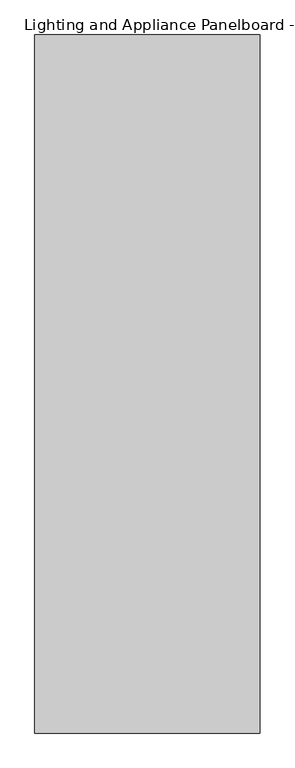
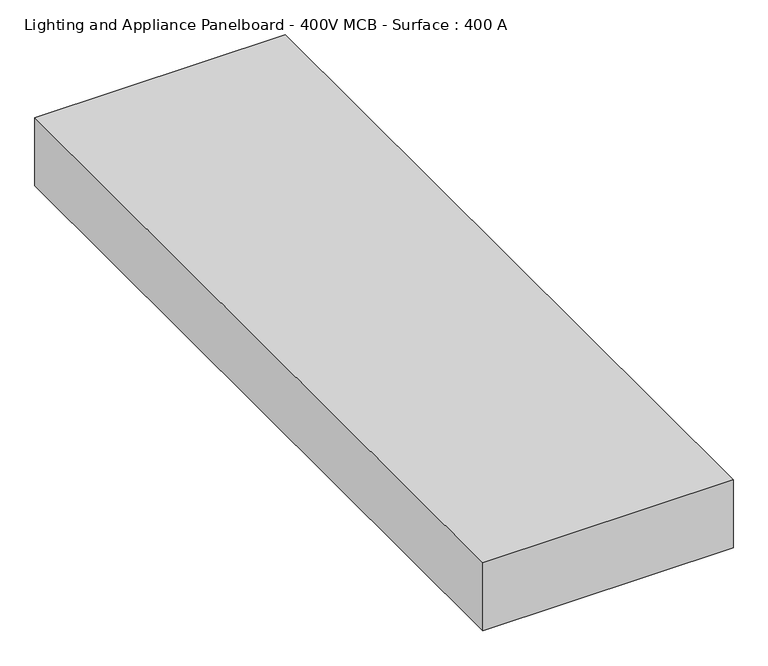
"""IFC4 building model written with IfcOpenShell, lengths in millimetres: proxy geometry, Lighting and Appliance Panelboard - 400V MCB - Surface : 400 A."""

import ifcopenshell
import ifcopenshell.guid

model = None  # the IFC model being written
_history = None  # IfcOwnerHistory: only IFC2X3 demands one
_inside = {}  # id of a spatial element -> (the spatial element, [elements in it])
_under = {}  # id of a project, library or spatial element -> (it, [spatial elements below it])
_declared = {}  # id of a project -> (the project, [libraries it declares])
_typed = {}  # id of a type object -> (the type object, [elements of that type])
_made_of = {}  # id of a material, layer set ... -> (it, [elements and type objects made of it])


def new_model(schema):
    """Start an empty IFC model of exactly this schema.

    Asked for "IFC4X3", IfcOpenShell would pick the latest addendum, in which some entities
    have other attributes; the version numbers below select the first issue.
    IFC2X3 requires an IfcOwnerHistory on every rooted entity: one is made here for all.
    """
    global model, _history
    if schema == "IFC4X3":
        model = ifcopenshell.file(schema_version=(4, 3, 0, 0))
    else:
        model = ifcopenshell.file(schema=schema)
    _inside.clear()
    _under.clear()
    _declared.clear()
    _typed.clear()
    _made_of.clear()
    _history = None
    if model.schema == "IFC2X3":
        org = make("IfcOrganization", Name="unknown")
        user = make(
            "IfcPersonAndOrganization",
            ThePerson=make("IfcPerson", FamilyName="unknown"),
            TheOrganization=org,
        )
        app = make(
            "IfcApplication",
            ApplicationDeveloper=org,
            Version="unknown",
            ApplicationFullName="unknown",
            ApplicationIdentifier="unknown",
        )
        _history = make(
            "IfcOwnerHistory",
            OwningUser=user,
            OwningApplication=app,
            ChangeAction="ADDED",
            CreationDate=0,
        )
    return model


def make(cls, **values):
    """One entity of the class cls with the attributes given. An attribute that is None is left unset."""
    return model.create_entity(
        cls, **{name: value for name, value in values.items() if value is not None}
    )


def rooted(cls, **values):
    """An entity with a GlobalId (a new one), such as an element, a storey or a relation."""
    return make(cls, GlobalId=ifcopenshell.guid.new(), OwnerHistory=_history, **values)


def si_unit(unit_type, name, prefix=None):
    """IfcSIUnit, for example si_unit("LENGTHUNIT", "METRE", prefix="MILLI")."""
    return make("IfcSIUnit", UnitType=unit_type, Prefix=prefix, Name=name)


def assignment(units):
    """IfcUnitAssignment: the units of a project."""
    return None if units is None else make("IfcUnitAssignment", Units=units)


def point(xyz):
    """IfcCartesianPoint."""
    return None if xyz is None else make("IfcCartesianPoint", Coordinates=xyz)


def direction(xyz):
    """IfcDirection."""
    return None if xyz is None else make("IfcDirection", DirectionRatios=xyz)


def frame(location, z_axis=None, x_axis=None):
    """IfcAxis2Placement3D, a coordinate frame: its origin and axes. An axis left out is left unset."""
    return make(
        "IfcAxis2Placement3D",
        Location=point(location),
        Axis=direction(z_axis),
        RefDirection=direction(x_axis),
    )


def origin():
    """The frame at (0, 0, 0) with its axes left unset."""
    return frame((0.0, 0.0, 0.0))


def origin_with_axes():
    """The frame at (0, 0, 0) with the z axis (0, 0, 1) and the x axis (1, 0, 0) written out."""
    return frame((0.0, 0.0, 0.0), z_axis=(0.0, 0.0, 1.0), x_axis=(1.0, 0.0, 0.0))


def place(relative_to, where):
    """IfcLocalPlacement: puts the frame where relative to a parent placement (None: the world)."""
    return make(
        "IfcLocalPlacement", PlacementRelTo=relative_to, RelativePlacement=where
    )


def context(
    kind, dimensions, precision=None, world=None, true_north=None, identifier=None
):
    """IfcGeometricRepresentationContext, for example the 3D "Model" context."""
    return make(
        "IfcGeometricRepresentationContext",
        ContextIdentifier=identifier,
        ContextType=kind,
        CoordinateSpaceDimension=dimensions,
        Precision=precision,
        WorldCoordinateSystem=world,
        TrueNorth=true_north,
    )


def project(units=None, contexts=None):
    """IfcProject with its units and contexts."""
    return rooted(
        "IfcProject",
        Name="project",
        RepresentationContexts=contexts,
        UnitsInContext=assignment(units),
    )


def spatial(cls, under=None, at=None, **own):
    """A site, building, storey or space (cls), placed at a placement, below another one or the project."""
    s = rooted(cls, ObjectPlacement=at, **own)
    if under is not None:
        _under.setdefault(under.id(), (under, []))[1].append(s)
    return s


def polyline(points):
    """IfcPolyline through the points."""
    return make("IfcPolyline", Points=[point(p) for p in points])


def outline(outer, holes=None, kind="AREA"):
    """IfcArbitraryClosedProfileDef: a profile drawn as a closed curve; with holes, ...WithVoids."""
    if holes is None:
        return make("IfcArbitraryClosedProfileDef", ProfileType=kind, OuterCurve=outer)
    return make(
        "IfcArbitraryProfileDefWithVoids",
        ProfileType=kind,
        OuterCurve=outer,
        InnerCurves=holes,
    )


def extrude(swept, where, along, depth):
    """IfcExtrudedAreaSolid: the profile swept, set in the frame where, extruded along a direction by depth."""
    return make(
        "IfcExtrudedAreaSolid",
        SweptArea=swept,
        Position=where,
        ExtrudedDirection=direction(along),
        Depth=depth,
    )


def shape(context_of_items, identifier, shape_type, items):
    """IfcShapeRepresentation: the items that make up one representation, for example the "Body"."""
    return make(
        "IfcShapeRepresentation",
        ContextOfItems=context_of_items,
        RepresentationIdentifier=identifier,
        RepresentationType=shape_type,
        Items=items,
    )


def source(mapping_origin, context_of_items, identifier, shape_type, items):
    """IfcRepresentationMap: a shape defined once, which mapped items show again and again."""
    return make(
        "IfcRepresentationMap",
        MappingOrigin=mapping_origin,
        MappedRepresentation=shape(context_of_items, identifier, shape_type, items),
    )


def transform(
    local_origin,
    x_axis=None,
    y_axis=None,
    z_axis=None,
    scale=None,
    scale2=None,
    scale3=None,
    uniform=True,
):
    """IfcCartesianTransformationOperator3D, or its non-uniform kind. x_axis, y_axis, z_axis: its Axis1, 2, 3."""
    if uniform:
        return make(
            "IfcCartesianTransformationOperator3D",
            Axis1=direction(x_axis),
            Axis2=direction(y_axis),
            LocalOrigin=point(local_origin),
            Scale=scale,
            Axis3=direction(z_axis),
        )
    return make(
        "IfcCartesianTransformationOperator3DnonUniform",
        Axis1=direction(x_axis),
        Axis2=direction(y_axis),
        LocalOrigin=point(local_origin),
        Scale=scale,
        Axis3=direction(z_axis),
        Scale2=scale2,
        Scale3=scale3,
    )


def mapped(mapping_source, mapping_target):
    """IfcMappedItem: shows the shape of a source again, moved by a transform."""
    return make(
        "IfcMappedItem", MappingSource=mapping_source, MappingTarget=mapping_target
    )


def made_of(thing, what):
    """Note that an element or type object is made of a material, layer set ...; save() writes the relation."""
    if what is not None:
        _made_of.setdefault(what.id(), (what, []))[1].append(thing)
    return thing


def element(
    cls,
    number,
    at=None,
    inside=None,
    cuts=None,
    type_object=None,
    material=None,
    context=None,
    identifier="Body",
    shape_type=None,
    held_by="IfcProductDefinitionShape",
    body=None,
    shapes=None,
    **own,
):
    """One element of the class cls, such as IfcWall. Its Tag is "e" and its number.

    at: its placement. inside: the storey or other place that contains it. cuts: it is an
    opening in that element (IfcRelVoidsElement). A single representation is given by context,
    identifier, shape_type and body (its items); several are given by shapes. held_by: the class
    of the entity that holds the representations. save() writes the other relations.
    """
    e = rooted(cls, Tag="e%d" % number, ObjectPlacement=at, **own)
    if body is not None:
        shapes = [shape(context, identifier, shape_type, body)]
    if shapes is not None:
        e.Representation = make(held_by, Representations=shapes)
    if inside is not None:
        _inside.setdefault(inside.id(), (inside, []))[1].append(e)
    if cuts is not None:
        rooted(
            "IfcRelVoidsElement", RelatingBuildingElement=cuts, RelatedOpeningElement=e
        )
    if type_object is not None:
        _typed.setdefault(type_object.id(), (type_object, []))[1].append(e)
    return made_of(e, material)


def aggregate(whole, parts):
    """IfcRelAggregates: a whole, such as a stair, and the parts it consists of."""
    return rooted("IfcRelAggregates", RelatingObject=whole, RelatedObjects=parts)


def save(model, path):
    """Write the relations noted so far, then the file.

    IfcRelAggregates (storeys below a building ...), IfcRelContainedInSpatialStructure (elements
    in a storey), IfcRelDefinesByType, IfcRelAssociatesMaterial and IfcRelDeclares: one each for
    every whole, place, type object, material and project.
    """
    for whole, parts in _under.values():
        aggregate(whole, parts)
    for where, things in _inside.values():
        rooted(
            "IfcRelContainedInSpatialStructure",
            RelatedElements=things,
            RelatingStructure=where,
        )
    for kind, things in _typed.values():
        rooted("IfcRelDefinesByType", RelatedObjects=things, RelatingType=kind)
    for what, things in _made_of.values():
        rooted("IfcRelAssociatesMaterial", RelatedObjects=things, RelatingMaterial=what)
    for by, libraries in _declared.values():
        rooted("IfcRelDeclares", RelatingContext=by, RelatedDefinitions=libraries)
    model.write(path)


def lighting_and_appliance_panelboard_400v_mcb_surface_400_a_826206d9(model_context):
    return source(origin(), model_context, "Body", "SweptSolid", [
        extrude(outline(polyline([(254.0, -1574.8), (-254.0, -1574.8), (-254.0, 0.0), (254.0, 0.0), (254.0, -1574.8)])), origin_with_axes(), (0.0, 0.0, 1.0), 146.1),
    ])


if __name__ == "__main__":
    model = new_model("IFC4")
    model_context = context("Model", 3, world=origin())
    ifc_project = project(units=[si_unit("LENGTHUNIT", "METRE", prefix="MILLI")], contexts=[model_context])
    site = spatial("IfcSite", under=ifc_project)
    building = spatial("IfcBuilding", under=site)
    placement = place(None, origin())
    lighting_and_appliance_panelboard_400v_mcb_surface_400_a_shape = lighting_and_appliance_panelboard_400v_mcb_surface_400_a_826206d9(model_context)
    element("IfcBuildingElementProxy", 1, Name="Lighting and Appliance Panelboard - 400V MCB - Surface : 400 A", ObjectType="Lighting and Appliance Panelboard - 400V MCB - Surface : 400 A", at=placement, inside=building, context=model_context, shape_type="MappedRepresentation", body=[
        mapped(lighting_and_appliance_panelboard_400v_mcb_surface_400_a_shape, transform((0.0, 0.0, 0.0), x_axis=(1.0, 0.0, 0.0), y_axis=(0.0, 1.0, 0.0), z_axis=(0.0, 0.0, 1.0))),
    ])
    save(model, "model.ifc")

# Revit data of these elements
# Type "Lighting and Appliance Panelboard - 400V MCB - Surface : 400 A"
#   Type Mark = "Lighting and Appliance Panelboard - 400V MCB - Surface"
#   Classification.OmniClass.21.Number = "21-04 50 30 50"
#   Classification.MasterFormat.Description = "Wiring Devices"
#   Classification.OmniClass.22.Number = "22-26 27 26"
#   Classification.OmniClass.21.Description = "Wiring Devices"
#   Classification.UniFormat.II.Description = "Wiring Devices"
#   Classification.MasterFormat.Number = "26 27 26"
#   Classification.OmniClass.23.Number = "23-35 31 29"
#   Classification.OmniClass.22.Description = "Wiring Devices"
#   Classification.OmniClass.23.Description = "Switchboards"
#   Classification.UniFormat.II.Number = "D5030.50"
#   COBie.Type.CreatedBy = "info@mma.ie"
#   COBie.Type.CreatedOn = "2017-07-25T10:15:16"
#   COBie.Type.Name = "Lighting and Appliance Panelboard - 400V MCB - Surface"
#   COBie.Type.Category = "23-35 31 29 : Switchboards"
#   COBie.Type.Description = "Lighting and Appliance Panelboard - 400V MCB - Surface_400 A"
#   COBie.Type.AssetType = "Fixed"
#   COBie.Type.Manufacturer = ""
#   COBie.Type.ModelNumber = ""
#   Wattage = "400"
#   Voltage = "600"
#   built-in parameter 1140081 [instance default] = "Surface"
#   Keynote = "26 24 16.A"
#   built-in parameter 1140083 [instance default] = "Type 1"
#   COBie.Type.ReplacementCost = 0
#   Width = 508 mm
#   built-in parameter 1140082 [instance default] = 100 (stored number, unit not read)
#   built-in parameter 1140140 [instance default] = 400 (stored number, unit not read)
#   L.A.P. Width = 508 mm
#   L.A.P. Height = 1574.8 mm
#   L.A.P. Depth = 146.1 mm
#   Height [instance default] = 1574.8 mm
#   Depth = 146.1 mm
#   Default Elevation = 1200 mm
#   Ballast Wattage = 400 W
#   Ballast Voltage = 600 V
#   42 Circuit Height = 1727.2 mm
#   30 Circuit Height = 1574.8 mm
#   18 Circuit Height = 1574.8 mm
#   12 Circuit Height = 1574.8 mm
#   COBie.Type = yes
#   built-in parameter 1140142 [instance default] = -1
#   built-in parameter 1140079 [instance default] = 12
#   built-in parameter 1155100 [instance default] = -1
#   Load Classification = Other
